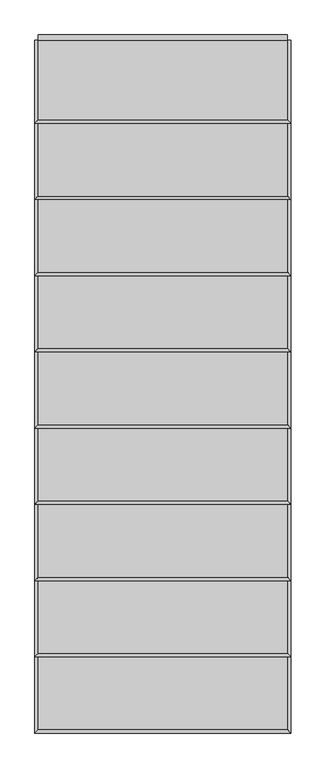
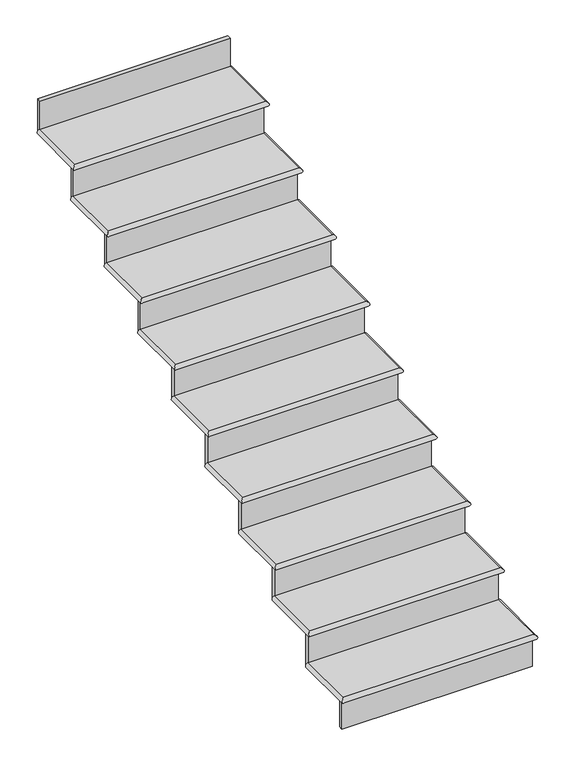
"""IFC4 building model written with IfcOpenShell, lengths in millimetres: stair flight geometry."""

from ifc_helpers import new_model, si_unit, frame, origin, place, context, project, spatial, circle_curve, ellipse_curve, faceted_brep, source, transform, mapped, element, save
from ifc_brep_helpers import plane_surface, cylinder_surface, advanced_brep


def stair_flight_efac3296(model_context):
    return source(origin(), model_context, "Body", "SolidModel", [
        advanced_brep(
        [(-6869.5581077, -11168.733999, 143.9333333), (-6869.5581077, -11168.733999, 169.3333333), (-7783.9581077, -11168.733999, 169.3333333), (-7783.9581077, -11168.733999, 143.9333333), (-6869.5581077, -10876.633999, 169.3333333), (-7783.9581077, -10876.633999, 169.3333333), (-7783.9581077, -10876.633999, 143.9333333), (-6869.5581077, -10876.633999, 143.9333333)],
        [
            (0, 1, ellipse_curve(frame((-6869.5581077, -11168.733999, 156.6333333), z_axis=(-0.7071067811865496, -0.7071067811865456, 0.0), x_axis=(0.7071067811865455, -0.7071067811865495, 0.0)), 17.9605122, 12.7)),
            (1, 2),
            (2, 3, ellipse_curve(frame((-7783.9581077, -11168.733999, 156.6333333), z_axis=(0.7071067811865455, -0.7071067811865495, 0.0), x_axis=(0.7071067811865496, 0.7071067811865455, 0.0)), 17.9605122, 12.7)),
            (3, 0),
            (4, 5),
            (5, 2),
            (1, 4),
            (6, 7),
            (7, 0),
            (3, 6),
            (4, 7, circle_curve(frame((-6869.5581077, -10876.633999, 156.6333333), z_axis=(0.0, 1.0, 0.0), x_axis=(-1.0, 0.0, 0.0)), 12.7)),
            (6, 5, circle_curve(frame((-7783.9581077, -10876.633999, 156.6333333), z_axis=(0.0, 1.0, 0.0), x_axis=(1.0, 0.0, 0.0)), 12.7)),
        ],
        [
            cylinder_surface(frame((-6869.5581077, -11168.733999, 156.6333333), z_axis=(1.0, 0.0, 0.0), x_axis=(0.0, 1.0, 0.0)), 12.7),
            plane_surface(frame((-7783.9581077, -10902.033999, 169.3333333), z_axis=(0.0, 0.0, 1.0), x_axis=(0.0, -1.0, 0.0))),
            plane_surface(frame((-7783.9581077, -10902.033999, 143.9333333), z_axis=(0.0, 0.0, -1.0), x_axis=(0.0, 1.0, 0.0))),
            plane_surface(frame((-6869.5581077, -10876.633999, 169.3333333), z_axis=(0.0, 1.0, 0.0), x_axis=(0.0, 0.0, -1.0))),
            cylinder_surface(frame((-6869.5581077, -10876.633999, 156.6333333), z_axis=(0.0, 1.0, 0.0), x_axis=(-1.0, 0.0, 0.0)), 12.7),
            cylinder_surface(frame((-7783.9581077, -11168.733999, 156.6333333), z_axis=(0.0, -1.0, 0.0), x_axis=(1.0, 0.0, 0.0)), 12.7),
        ],
        [
            (0, [[1, 2, 3, 4]]),
            (1, [[5, 6, -2, 7]]),
            (2, [[8, 9, -4, 10]]),
            (3, [[-5, 11, -8, 12]]),
            (4, [[-11, -7, -1, -9]]),
            (5, [[-3, -6, -12, -10]]),
        ],
    ),
        faceted_brep([(-6869.5581077, -11156.033999, 143.9333333), (-6869.5581077, -11156.033999, 0.0), (-6869.5581077, -11136.983999, 0.0), (-6869.5581077, -11136.983999, 143.9333333), (-7783.9581077, -11156.033999, 143.9333333), (-7783.9581077, -11136.983999, 143.9333333), (-7783.9581077, -11136.983999, 0.0), (-7783.9581077, -11156.033999, 0.0)], [[[0, 1, 2, 3]], [[4, 5, 6, 7]], [[1, 0, 4, 7]], [[2, 1, 7, 6]], [[3, 2, 6, 5]], [[0, 3, 5, 4]]]),
        faceted_brep([(-6869.5581077, -10876.633999, 313.2666667), (-6869.5581077, -10876.633999, 143.9333333), (-6869.5581077, -10857.583999, 143.9333333), (-6869.5581077, -10857.583999, 313.2666667), (-7783.9581077, -10876.633999, 313.2666667), (-7783.9581077, -10857.583999, 313.2666667), (-7783.9581077, -10857.583999, 143.9333333), (-7783.9581077, -10876.633999, 143.9333333)], [[[0, 1, 2, 3]], [[4, 5, 6, 7]], [[1, 0, 4, 7]], [[2, 1, 7, 6]], [[3, 2, 6, 5]], [[0, 3, 5, 4]]]),
        advanced_brep(
        [(-6869.5581077, -10597.233999, 338.6666667), (-7783.9581077, -10597.233999, 338.6666667), (-7783.9581077, -10889.333999, 338.6666667), (-6869.5581077, -10889.333999, 338.6666667), (-7783.9581077, -10597.233999, 313.2666667), (-6869.5581077, -10597.233999, 313.2666667), (-6869.5581077, -10889.333999, 313.2666667), (-7783.9581077, -10889.333999, 313.2666667)],
        [
            (0, 1),
            (1, 2),
            (2, 3),
            (3, 0),
            (4, 5),
            (5, 6),
            (6, 7),
            (7, 4),
            (0, 5, circle_curve(frame((-6869.5581077, -10597.233999, 325.9666667), z_axis=(0.0, 1.0, 0.0), x_axis=(-1.0, 0.0, 0.0)), 12.7)),
            (4, 1, circle_curve(frame((-7783.9581077, -10597.233999, 325.9666667), z_axis=(0.0, 1.0, 0.0), x_axis=(1.0, 0.0, 0.0)), 12.7)),
            (6, 3, ellipse_curve(frame((-6869.5581077, -10889.333999, 325.9666667), z_axis=(-0.7071067811865481, -0.7071067811865469, 0.0), x_axis=(0.7071067811865469, -0.7071067811865481, 0.0)), 17.9605122, 12.7)),
            (2, 7, ellipse_curve(frame((-7783.9581077, -10889.333999, 325.9666667), z_axis=(0.7071067811865469, -0.7071067811865481, 0.0), x_axis=(0.7071067811865481, 0.7071067811865468, 0.0)), 17.9605122, 12.7)),
        ],
        [
            plane_surface(frame((-7783.9581077, -10902.033999, 338.6666667), z_axis=(0.0, 0.0, 1.0), x_axis=(0.0, -1.0, 0.0))),
            plane_surface(frame((-7783.9581077, -10902.033999, 313.2666667), z_axis=(0.0, 0.0, -1.0), x_axis=(0.0, 1.0, 0.0))),
            plane_surface(frame((-6869.5581077, -10597.233999, 338.6666667), z_axis=(0.0, 1.0, 0.0), x_axis=(0.0, 0.0, -1.0))),
            cylinder_surface(frame((-6869.5581077, -10889.333999, 325.9666667), z_axis=(1.0, 0.0, 0.0), x_axis=(0.0, 1.0, 0.0)), 12.7),
            cylinder_surface(frame((-6869.5581077, -10597.233999, 325.9666667), z_axis=(0.0, 1.0, 0.0), x_axis=(-1.0, 0.0, 0.0)), 12.7),
            cylinder_surface(frame((-7783.9581077, -10889.333999, 325.9666667), z_axis=(0.0, -1.0, 0.0), x_axis=(1.0, 0.0, 0.0)), 12.7),
        ],
        [
            (0, [[1, 2, 3, 4]]),
            (1, [[5, 6, 7, 8]]),
            (2, [[-1, 9, -5, 10]]),
            (3, [[11, -3, 12, -7]]),
            (4, [[-9, -4, -11, -6]]),
            (5, [[-12, -2, -10, -8]]),
        ],
    ),
        faceted_brep([(-6869.5581077, -10597.233999, 482.6), (-6869.5581077, -10597.233999, 313.2666667), (-6869.5581077, -10578.183999, 313.2666667), (-6869.5581077, -10578.183999, 482.6), (-7783.9581077, -10597.233999, 482.6), (-7783.9581077, -10578.183999, 482.6), (-7783.9581077, -10578.183999, 313.2666667), (-7783.9581077, -10597.233999, 313.2666667)], [[[0, 1, 2, 3]], [[4, 5, 6, 7]], [[1, 0, 4, 7]], [[2, 1, 7, 6]], [[3, 2, 6, 5]], [[0, 3, 5, 4]]]),
        advanced_brep(
        [(-6869.5581077, -10317.833999, 508.0), (-7783.9581077, -10317.833999, 508.0), (-7783.9581077, -10609.933999, 508.0), (-6869.5581077, -10609.933999, 508.0), (-7783.9581077, -10317.833999, 482.6), (-6869.5581077, -10317.833999, 482.6), (-6869.5581077, -10609.933999, 482.6), (-7783.9581077, -10609.933999, 482.6)],
        [
            (0, 1),
            (1, 2),
            (2, 3),
            (3, 0),
            (4, 5),
            (5, 6),
            (6, 7),
            (7, 4),
            (0, 5, circle_curve(frame((-6869.5581077, -10317.833999, 495.3), z_axis=(0.0, 1.0, 0.0), x_axis=(-1.0, 0.0, 0.0)), 12.7)),
            (4, 1, circle_curve(frame((-7783.9581077, -10317.833999, 495.3), z_axis=(0.0, 1.0, 0.0), x_axis=(1.0, 0.0, 0.0)), 12.7)),
            (6, 3, ellipse_curve(frame((-6869.5581077, -10609.933999, 495.3), z_axis=(-0.7071067811865481, -0.7071067811865469, 0.0), x_axis=(0.7071067811865469, -0.7071067811865481, 0.0)), 17.9605122, 12.7)),
            (2, 7, ellipse_curve(frame((-7783.9581077, -10609.933999, 495.3), z_axis=(0.7071067811865469, -0.7071067811865481, 0.0), x_axis=(0.7071067811865481, 0.7071067811865468, 0.0)), 17.9605122, 12.7)),
        ],
        [
            plane_surface(frame((-7783.9581077, -10622.633999, 508.0), z_axis=(0.0, 0.0, 1.0), x_axis=(0.0, -1.0, 0.0))),
            plane_surface(frame((-7783.9581077, -10622.633999, 482.6), z_axis=(0.0, 0.0, -1.0), x_axis=(0.0, 1.0, 0.0))),
            plane_surface(frame((-6869.5581077, -10317.833999, 508.0), z_axis=(0.0, 1.0, 0.0), x_axis=(0.0, 0.0, -1.0))),
            cylinder_surface(frame((-6869.5581077, -10609.933999, 495.3), z_axis=(1.0, 0.0, 0.0), x_axis=(0.0, 1.0, 0.0)), 12.7),
            cylinder_surface(frame((-6869.5581077, -10317.833999, 495.3), z_axis=(0.0, 1.0, 0.0), x_axis=(-1.0, 0.0, 0.0)), 12.7),
            cylinder_surface(frame((-7783.9581077, -10609.933999, 495.3), z_axis=(0.0, -1.0, 0.0), x_axis=(1.0, 0.0, 0.0)), 12.7),
        ],
        [
            (0, [[1, 2, 3, 4]]),
            (1, [[5, 6, 7, 8]]),
            (2, [[-1, 9, -5, 10]]),
            (3, [[11, -3, 12, -7]]),
            (4, [[-9, -4, -11, -6]]),
            (5, [[-12, -2, -10, -8]]),
        ],
    ),
        faceted_brep([(-6869.5581077, -10317.833999, 651.9333333), (-6869.5581077, -10317.833999, 482.6), (-6869.5581077, -10298.783999, 482.6), (-6869.5581077, -10298.783999, 651.9333333), (-7783.9581077, -10317.833999, 651.9333333), (-7783.9581077, -10298.783999, 651.9333333), (-7783.9581077, -10298.783999, 482.6), (-7783.9581077, -10317.833999, 482.6)], [[[0, 1, 2, 3]], [[4, 5, 6, 7]], [[1, 0, 4, 7]], [[2, 1, 7, 6]], [[3, 2, 6, 5]], [[0, 3, 5, 4]]]),
        advanced_brep(
        [(-6869.5581077, -10038.433999, 677.3333333), (-7783.9581077, -10038.433999, 677.3333333), (-7783.9581077, -10330.533999, 677.3333333), (-6869.5581077, -10330.533999, 677.3333333), (-7783.9581077, -10038.433999, 651.9333333), (-6869.5581077, -10038.433999, 651.9333333), (-6869.5581077, -10330.533999, 651.9333333), (-7783.9581077, -10330.533999, 651.9333333)],
        [
            (0, 1),
            (1, 2),
            (2, 3),
            (3, 0),
            (4, 5),
            (5, 6),
            (6, 7),
            (7, 4),
            (0, 5, circle_curve(frame((-6869.5581077, -10038.433999, 664.6333333), z_axis=(0.0, 1.0, 0.0), x_axis=(-1.0, 0.0, 0.0)), 12.7)),
            (4, 1, circle_curve(frame((-7783.9581077, -10038.433999, 664.6333333), z_axis=(0.0, 1.0, 0.0), x_axis=(1.0, 0.0, 0.0)), 12.7)),
            (6, 3, ellipse_curve(frame((-6869.5581077, -10330.533999, 664.6333333), z_axis=(-0.7071067811865481, -0.7071067811865469, 0.0), x_axis=(0.7071067811865469, -0.7071067811865481, 0.0)), 17.9605122, 12.7)),
            (2, 7, ellipse_curve(frame((-7783.9581077, -10330.533999, 664.6333333), z_axis=(0.7071067811865469, -0.7071067811865481, 0.0), x_axis=(0.7071067811865481, 0.7071067811865468, 0.0)), 17.9605122, 12.7)),
        ],
        [
            plane_surface(frame((-7783.9581077, -10343.233999, 677.3333333), z_axis=(0.0, 0.0, 1.0), x_axis=(0.0, -1.0, 0.0))),
            plane_surface(frame((-7783.9581077, -10343.233999, 651.9333333), z_axis=(0.0, 0.0, -1.0), x_axis=(0.0, 1.0, 0.0))),
            plane_surface(frame((-6869.5581077, -10038.433999, 677.3333333), z_axis=(0.0, 1.0, 0.0), x_axis=(0.0, 0.0, -1.0))),
            cylinder_surface(frame((-6869.5581077, -10330.533999, 664.6333333), z_axis=(1.0, 0.0, 0.0), x_axis=(0.0, 1.0, 0.0)), 12.7),
            cylinder_surface(frame((-6869.5581077, -10038.433999, 664.6333333), z_axis=(0.0, 1.0, 0.0), x_axis=(-1.0, 0.0, 0.0)), 12.7),
            cylinder_surface(frame((-7783.9581077, -10330.533999, 664.6333333), z_axis=(0.0, -1.0, 0.0), x_axis=(1.0, 0.0, 0.0)), 12.7),
        ],
        [
            (0, [[1, 2, 3, 4]]),
            (1, [[5, 6, 7, 8]]),
            (2, [[-1, 9, -5, 10]]),
            (3, [[11, -3, 12, -7]]),
            (4, [[-9, -4, -11, -6]]),
            (5, [[-12, -2, -10, -8]]),
        ],
    ),
        faceted_brep([(-6869.5581077, -10038.433999, 821.2666667), (-6869.5581077, -10038.433999, 651.9333333), (-6869.5581077, -10019.383999, 651.9333333), (-6869.5581077, -10019.383999, 821.2666667), (-7783.9581077, -10038.433999, 821.2666667), (-7783.9581077, -10019.383999, 821.2666667), (-7783.9581077, -10019.383999, 651.9333333), (-7783.9581077, -10038.433999, 651.9333333)], [[[0, 1, 2, 3]], [[4, 5, 6, 7]], [[1, 0, 4, 7]], [[2, 1, 7, 6]], [[3, 2, 6, 5]], [[0, 3, 5, 4]]]),
        advanced_brep(
        [(-6869.5581077, -9759.033999, 846.6666667), (-7783.9581077, -9759.033999, 846.6666667), (-7783.9581077, -10051.133999, 846.6666667), (-6869.5581077, -10051.133999, 846.6666667), (-7783.9581077, -9759.033999, 821.2666667), (-6869.5581077, -9759.033999, 821.2666667), (-6869.5581077, -10051.133999, 821.2666667), (-7783.9581077, -10051.133999, 821.2666667)],
        [
            (0, 1),
            (1, 2),
            (2, 3),
            (3, 0),
            (4, 5),
            (5, 6),
            (6, 7),
            (7, 4),
            (0, 5, circle_curve(frame((-6869.5581077, -9759.033999, 833.9666667), z_axis=(0.0, 1.0, 0.0), x_axis=(-1.0, 0.0, 0.0)), 12.7)),
            (4, 1, circle_curve(frame((-7783.9581077, -9759.033999, 833.9666667), z_axis=(0.0, 1.0, 0.0), x_axis=(1.0, 0.0, 0.0)), 12.7)),
            (6, 3, ellipse_curve(frame((-6869.5581077, -10051.133999, 833.9666667), z_axis=(-0.7071067811865481, -0.7071067811865469, 0.0), x_axis=(0.7071067811865469, -0.7071067811865481, 0.0)), 17.9605122, 12.7)),
            (2, 7, ellipse_curve(frame((-7783.9581077, -10051.133999, 833.9666667), z_axis=(0.7071067811865469, -0.7071067811865481, 0.0), x_axis=(0.7071067811865481, 0.7071067811865468, 0.0)), 17.9605122, 12.7)),
        ],
        [
            plane_surface(frame((-7783.9581077, -10063.833999, 846.6666667), z_axis=(0.0, 0.0, 1.0), x_axis=(0.0, -1.0, 0.0))),
            plane_surface(frame((-7783.9581077, -10063.833999, 821.2666667), z_axis=(0.0, 0.0, -1.0), x_axis=(0.0, 1.0, 0.0))),
            plane_surface(frame((-6869.5581077, -9759.033999, 846.6666667), z_axis=(0.0, 1.0, 0.0), x_axis=(0.0, 0.0, -1.0))),
            cylinder_surface(frame((-6869.5581077, -10051.133999, 833.9666667), z_axis=(1.0, 0.0, 0.0), x_axis=(0.0, 1.0, 0.0)), 12.7),
            cylinder_surface(frame((-6869.5581077, -9759.033999, 833.9666667), z_axis=(0.0, 1.0, 0.0), x_axis=(-1.0, 0.0, 0.0)), 12.7),
            cylinder_surface(frame((-7783.9581077, -10051.133999, 833.9666667), z_axis=(0.0, -1.0, 0.0), x_axis=(1.0, 0.0, 0.0)), 12.7),
        ],
        [
            (0, [[1, 2, 3, 4]]),
            (1, [[5, 6, 7, 8]]),
            (2, [[-1, 9, -5, 10]]),
            (3, [[11, -3, 12, -7]]),
            (4, [[-9, -4, -11, -6]]),
            (5, [[-12, -2, -10, -8]]),
        ],
    ),
        faceted_brep([(-6869.5581077, -9759.033999, 990.6), (-6869.5581077, -9759.033999, 821.2666667), (-6869.5581077, -9739.983999, 821.2666667), (-6869.5581077, -9739.983999, 990.6), (-7783.9581077, -9759.033999, 990.6), (-7783.9581077, -9739.983999, 990.6), (-7783.9581077, -9739.983999, 821.2666667), (-7783.9581077, -9759.033999, 821.2666667)], [[[0, 1, 2, 3]], [[4, 5, 6, 7]], [[1, 0, 4, 7]], [[2, 1, 7, 6]], [[3, 2, 6, 5]], [[0, 3, 5, 4]]]),
        advanced_brep(
        [(-6869.5581077, -9479.633999, 1016.0), (-7783.9581077, -9479.633999, 1016.0), (-7783.9581077, -9771.733999, 1016.0), (-6869.5581077, -9771.733999, 1016.0), (-7783.9581077, -9479.633999, 990.6), (-6869.5581077, -9479.633999, 990.6), (-6869.5581077, -9771.733999, 990.6), (-7783.9581077, -9771.733999, 990.6)],
        [
            (0, 1),
            (1, 2),
            (2, 3),
            (3, 0),
            (4, 5),
            (5, 6),
            (6, 7),
            (7, 4),
            (0, 5, circle_curve(frame((-6869.5581077, -9479.633999, 1003.3), z_axis=(0.0, 1.0, 0.0), x_axis=(-1.0, 0.0, 0.0)), 12.7)),
            (4, 1, circle_curve(frame((-7783.9581077, -9479.633999, 1003.3), z_axis=(0.0, 1.0, 0.0), x_axis=(1.0, 0.0, 0.0)), 12.7)),
            (6, 3, ellipse_curve(frame((-6869.5581077, -9771.733999, 1003.3), z_axis=(-0.7071067811865481, -0.7071067811865469, 0.0), x_axis=(0.7071067811865469, -0.7071067811865481, 0.0)), 17.9605122, 12.7)),
            (2, 7, ellipse_curve(frame((-7783.9581077, -9771.733999, 1003.3), z_axis=(0.7071067811865469, -0.7071067811865481, 0.0), x_axis=(0.7071067811865481, 0.7071067811865468, 0.0)), 17.9605122, 12.7)),
        ],
        [
            plane_surface(frame((-7783.9581077, -9784.433999, 1016.0), z_axis=(0.0, 0.0, 1.0), x_axis=(0.0, -1.0, 0.0))),
            plane_surface(frame((-7783.9581077, -9784.433999, 990.6), z_axis=(0.0, 0.0, -1.0), x_axis=(0.0, 1.0, 0.0))),
            plane_surface(frame((-6869.5581077, -9479.633999, 1016.0), z_axis=(0.0, 1.0, 0.0), x_axis=(0.0, 0.0, -1.0))),
            cylinder_surface(frame((-6869.5581077, -9771.733999, 1003.3), z_axis=(1.0, 0.0, 0.0), x_axis=(0.0, 1.0, 0.0)), 12.7),
            cylinder_surface(frame((-6869.5581077, -9479.633999, 1003.3), z_axis=(0.0, 1.0, 0.0), x_axis=(-1.0, 0.0, 0.0)), 12.7),
            cylinder_surface(frame((-7783.9581077, -9771.733999, 1003.3), z_axis=(0.0, -1.0, 0.0), x_axis=(1.0, 0.0, 0.0)), 12.7),
        ],
        [
            (0, [[1, 2, 3, 4]]),
            (1, [[5, 6, 7, 8]]),
            (2, [[-1, 9, -5, 10]]),
            (3, [[11, -3, 12, -7]]),
            (4, [[-9, -4, -11, -6]]),
            (5, [[-12, -2, -10, -8]]),
        ],
    ),
        faceted_brep([(-6869.5581077, -9479.633999, 1159.9333333), (-6869.5581077, -9479.633999, 990.6), (-6869.5581077, -9460.583999, 990.6), (-6869.5581077, -9460.583999, 1159.9333333), (-7783.9581077, -9479.633999, 1159.9333333), (-7783.9581077, -9460.583999, 1159.9333333), (-7783.9581077, -9460.583999, 990.6), (-7783.9581077, -9479.633999, 990.6)], [[[0, 1, 2, 3]], [[4, 5, 6, 7]], [[1, 0, 4, 7]], [[2, 1, 7, 6]], [[3, 2, 6, 5]], [[0, 3, 5, 4]]]),
        advanced_brep(
        [(-6869.5581077, -9200.233999, 1185.3333333), (-7783.9581077, -9200.233999, 1185.3333333), (-7783.9581077, -9492.333999, 1185.3333333), (-6869.5581077, -9492.333999, 1185.3333333), (-7783.9581077, -9200.233999, 1159.9333333), (-6869.5581077, -9200.233999, 1159.9333333), (-6869.5581077, -9492.333999, 1159.9333333), (-7783.9581077, -9492.333999, 1159.9333333)],
        [
            (0, 1),
            (1, 2),
            (2, 3),
            (3, 0),
            (4, 5),
            (5, 6),
            (6, 7),
            (7, 4),
            (0, 5, circle_curve(frame((-6869.5581077, -9200.233999, 1172.6333333), z_axis=(0.0, 1.0, 0.0), x_axis=(-1.0, 0.0, 0.0)), 12.7)),
            (4, 1, circle_curve(frame((-7783.9581077, -9200.233999, 1172.6333333), z_axis=(0.0, 1.0, 0.0), x_axis=(1.0, 0.0, 0.0)), 12.7)),
            (6, 3, ellipse_curve(frame((-6869.5581077, -9492.333999, 1172.6333333), z_axis=(-0.7071067811865481, -0.7071067811865469, 0.0), x_axis=(0.7071067811865469, -0.7071067811865481, 0.0)), 17.9605122, 12.7)),
            (2, 7, ellipse_curve(frame((-7783.9581077, -9492.333999, 1172.6333333), z_axis=(0.7071067811865469, -0.7071067811865481, 0.0), x_axis=(0.7071067811865481, 0.7071067811865468, 0.0)), 17.9605122, 12.7)),
        ],
        [
            plane_surface(frame((-7783.9581077, -9505.033999, 1185.3333333), z_axis=(0.0, 0.0, 1.0), x_axis=(0.0, -1.0, 0.0))),
            plane_surface(frame((-7783.9581077, -9505.033999, 1159.9333333), z_axis=(0.0, 0.0, -1.0), x_axis=(0.0, 1.0, 0.0))),
            plane_surface(frame((-6869.5581077, -9200.233999, 1185.3333333), z_axis=(0.0, 1.0, 0.0), x_axis=(0.0, 0.0, -1.0))),
            cylinder_surface(frame((-6869.5581077, -9492.333999, 1172.6333333), z_axis=(1.0, 0.0, 0.0), x_axis=(0.0, 1.0, 0.0)), 12.7),
            cylinder_surface(frame((-6869.5581077, -9200.233999, 1172.6333333), z_axis=(0.0, 1.0, 0.0), x_axis=(-1.0, 0.0, 0.0)), 12.7),
            cylinder_surface(frame((-7783.9581077, -9492.333999, 1172.6333333), z_axis=(0.0, -1.0, 0.0), x_axis=(1.0, 0.0, 0.0)), 12.7),
        ],
        [
            (0, [[1, 2, 3, 4]]),
            (1, [[5, 6, 7, 8]]),
            (2, [[-1, 9, -5, 10]]),
            (3, [[11, -3, 12, -7]]),
            (4, [[-9, -4, -11, -6]]),
            (5, [[-12, -2, -10, -8]]),
        ],
    ),
        faceted_brep([(-6869.5581077, -9200.233999, 1329.2666667), (-6869.5581077, -9200.233999, 1159.9333333), (-6869.5581077, -9181.183999, 1159.9333333), (-6869.5581077, -9181.183999, 1329.2666667), (-7783.9581077, -9200.233999, 1329.2666667), (-7783.9581077, -9181.183999, 1329.2666667), (-7783.9581077, -9181.183999, 1159.9333333), (-7783.9581077, -9200.233999, 1159.9333333)], [[[0, 1, 2, 3]], [[4, 5, 6, 7]], [[1, 0, 4, 7]], [[2, 1, 7, 6]], [[3, 2, 6, 5]], [[0, 3, 5, 4]]]),
        advanced_brep(
        [(-6869.5581077, -8920.833999, 1354.6666667), (-7783.9581077, -8920.833999, 1354.6666667), (-7783.9581077, -9212.933999, 1354.6666667), (-6869.5581077, -9212.933999, 1354.6666667), (-7783.9581077, -8920.833999, 1329.2666667), (-6869.5581077, -8920.833999, 1329.2666667), (-6869.5581077, -9212.933999, 1329.2666667), (-7783.9581077, -9212.933999, 1329.2666667)],
        [
            (0, 1),
            (1, 2),
            (2, 3),
            (3, 0),
            (4, 5),
            (5, 6),
            (6, 7),
            (7, 4),
            (0, 5, circle_curve(frame((-6869.5581077, -8920.833999, 1341.9666667), z_axis=(0.0, 1.0, 0.0), x_axis=(-1.0, 0.0, 0.0)), 12.7)),
            (4, 1, circle_curve(frame((-7783.9581077, -8920.833999, 1341.9666667), z_axis=(0.0, 1.0, 0.0), x_axis=(1.0, 0.0, 0.0)), 12.7)),
            (6, 3, ellipse_curve(frame((-6869.5581077, -9212.933999, 1341.9666667), z_axis=(-0.7071067811865481, -0.7071067811865469, 0.0), x_axis=(0.7071067811865469, -0.7071067811865481, 0.0)), 17.9605122, 12.7)),
            (2, 7, ellipse_curve(frame((-7783.9581077, -9212.933999, 1341.9666667), z_axis=(0.7071067811865469, -0.7071067811865481, 0.0), x_axis=(0.7071067811865481, 0.7071067811865468, 0.0)), 17.9605122, 12.7)),
        ],
        [
            plane_surface(frame((-7783.9581077, -9225.633999, 1354.6666667), z_axis=(0.0, 0.0, 1.0), x_axis=(0.0, -1.0, 0.0))),
            plane_surface(frame((-7783.9581077, -9225.633999, 1329.2666667), z_axis=(0.0, 0.0, -1.0), x_axis=(0.0, 1.0, 0.0))),
            plane_surface(frame((-6869.5581077, -8920.833999, 1354.6666667), z_axis=(0.0, 1.0, 0.0), x_axis=(0.0, 0.0, -1.0))),
            cylinder_surface(frame((-6869.5581077, -9212.933999, 1341.9666667), z_axis=(1.0, 0.0, 0.0), x_axis=(0.0, 1.0, 0.0)), 12.7),
            cylinder_surface(frame((-6869.5581077, -8920.833999, 1341.9666667), z_axis=(0.0, 1.0, 0.0), x_axis=(-1.0, 0.0, 0.0)), 12.7),
            cylinder_surface(frame((-7783.9581077, -9212.933999, 1341.9666667), z_axis=(0.0, -1.0, 0.0), x_axis=(1.0, 0.0, 0.0)), 12.7),
        ],
        [
            (0, [[1, 2, 3, 4]]),
            (1, [[5, 6, 7, 8]]),
            (2, [[-1, 9, -5, 10]]),
            (3, [[11, -3, 12, -7]]),
            (4, [[-9, -4, -11, -6]]),
            (5, [[-12, -2, -10, -8]]),
        ],
    ),
        faceted_brep([(-6869.5581077, -8641.433999, 1667.9333333), (-6869.5581077, -8641.433999, 1498.6), (-6869.5581077, -8622.383999, 1498.6), (-6869.5581077, -8622.383999, 1667.9333333), (-7783.9581077, -8641.433999, 1667.9333333), (-7783.9581077, -8622.383999, 1667.9333333), (-7783.9581077, -8622.383999, 1498.6), (-7783.9581077, -8641.433999, 1498.6)], [[[0, 1, 2, 3]], [[4, 5, 6, 7]], [[1, 0, 4, 7]], [[2, 1, 7, 6]], [[3, 2, 6, 5]], [[0, 3, 5, 4]]]),
        faceted_brep([(-6869.5581077, -8920.833999, 1498.6), (-6869.5581077, -8920.833999, 1329.2666667), (-6869.5581077, -8901.783999, 1329.2666667), (-6869.5581077, -8901.783999, 1498.6), (-7783.9581077, -8920.833999, 1498.6), (-7783.9581077, -8901.783999, 1498.6), (-7783.9581077, -8901.783999, 1329.2666667), (-7783.9581077, -8920.833999, 1329.2666667)], [[[0, 1, 2, 3]], [[4, 5, 6, 7]], [[1, 0, 4, 7]], [[2, 1, 7, 6]], [[3, 2, 6, 5]], [[0, 3, 5, 4]]]),
        advanced_brep(
        [(-6869.5581077, -8641.433999, 1524.0), (-7783.9581077, -8641.433999, 1524.0), (-7783.9581077, -8666.833999, 1524.0), (-7783.9581077, -8933.533999, 1524.0), (-6869.5581077, -8933.533999, 1524.0), (-6869.5581077, -8666.833999, 1524.0), (-7783.9581077, -8641.433999, 1498.6), (-6869.5581077, -8641.433999, 1498.6), (-6869.5581077, -8666.833999, 1498.6), (-6869.5581077, -8933.533999, 1498.6), (-7783.9581077, -8933.533999, 1498.6), (-7783.9581077, -8666.833999, 1498.6)],
        [
            (0, 1),
            (1, 2),
            (2, 3),
            (3, 4),
            (4, 5),
            (5, 0),
            (6, 7),
            (7, 8),
            (8, 9),
            (9, 10),
            (10, 11),
            (11, 6),
            (0, 7, circle_curve(frame((-6869.5581077, -8641.433999, 1511.3), z_axis=(0.0, 1.0, 0.0), x_axis=(-1.0, 0.0, 0.0)), 12.7)),
            (6, 1, circle_curve(frame((-7783.9581077, -8641.433999, 1511.3), z_axis=(0.0, 1.0, 0.0), x_axis=(1.0, 0.0, 0.0)), 12.7)),
            (9, 4, ellipse_curve(frame((-6869.5581077, -8933.533999, 1511.3), z_axis=(-0.7071067811865475, -0.7071067811865475, 0.0), x_axis=(0.7071067811865476, -0.7071067811865474, 0.0)), 17.9605122, 12.7)),
            (3, 10, ellipse_curve(frame((-7783.9581077, -8933.533999, 1511.3), z_axis=(0.7071067811865469, -0.7071067811865481, 0.0), x_axis=(0.7071067811865481, 0.7071067811865469, 0.0)), 17.9605122, 12.7)),
        ],
        [
            plane_surface(frame((-7783.9581077, -8666.833999, 1524.0), z_axis=(0.0, 0.0, 1.0), x_axis=(0.0, -1.0, 0.0))),
            plane_surface(frame((-7783.9581077, -8666.833999, 1498.6), z_axis=(0.0, 0.0, -1.0), x_axis=(0.0, 1.0, 0.0))),
            plane_surface(frame((-6869.5581077, -8641.433999, 1524.0), z_axis=(0.0, 1.0, 0.0), x_axis=(0.0, 0.0, -1.0))),
            cylinder_surface(frame((-6869.5581077, -8933.533999, 1511.3), z_axis=(1.0, 0.0, 0.0), x_axis=(0.0, 1.0, 0.0)), 12.7),
            cylinder_surface(frame((-6869.5581077, -8641.433999, 1511.3), z_axis=(0.0, 1.0, 0.0), x_axis=(-1.0, 0.0, 0.0)), 12.7),
            cylinder_surface(frame((-7783.9581077, -8933.533999, 1511.3), z_axis=(0.0, -1.0, 0.0), x_axis=(1.0, 0.0, 0.0)), 12.7),
        ],
        [
            (0, [[1, 2, 3, 4, 5, 6]]),
            (1, [[7, 8, 9, 10, 11, 12]]),
            (2, [[-1, 13, -7, 14]]),
            (3, [[15, -4, 16, -10]]),
            (4, [[-13, -6, -5, -15, -9, -8]]),
            (5, [[-16, -3, -2, -14, -12, -11]]),
        ],
    ),
    ])


if __name__ == "__main__":
    model = new_model("IFC4")
    model_context = context("Model", 3, world=origin())
    ifc_project = project(units=[si_unit("LENGTHUNIT", "METRE", prefix="MILLI")], contexts=[model_context])
    site = spatial("IfcSite", under=ifc_project)
    building = spatial("IfcBuilding", under=site)
    placement = place(None, origin())
    stair_flight_shape = stair_flight_efac3296(model_context)
    element("IfcStairFlight", 1, at=placement, inside=building, context=model_context, shape_type="MappedRepresentation", body=[
        mapped(stair_flight_shape, transform((0.0, 0.0, 0.0), x_axis=(1.0, 0.0, 0.0), y_axis=(0.0, 1.0, 0.0), z_axis=(0.0, 0.0, 1.0))),
    ])
    save(model, "model.ifc")

# Revit data of these elements
# Element 1 (IfcStairFlight)
#   Materials on its faces: "Wood - Cherry"
# Materials
#   "Wood - Cherry": class "Unassigned", colour RGB 226 177 128, transparency 0
